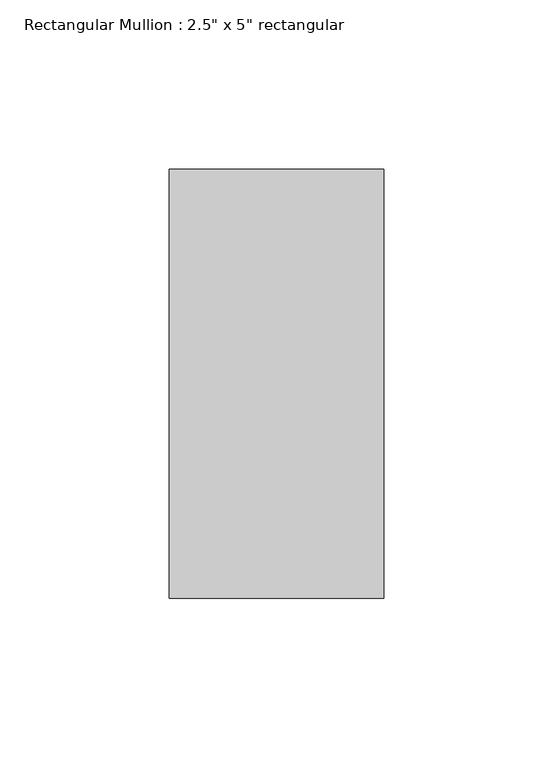
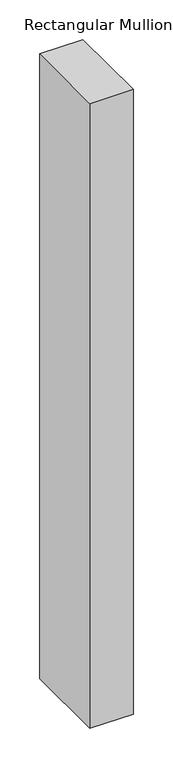
"""IFC4 building model written with IfcOpenShell, lengths in millimetres: member geometry."""

import ifcopenshell
import ifcopenshell.guid

model = None  # the IFC model being written
_history = None  # IfcOwnerHistory: only IFC2X3 demands one
_inside = {}  # id of a spatial element -> (the spatial element, [elements in it])
_under = {}  # id of a project, library or spatial element -> (it, [spatial elements below it])
_declared = {}  # id of a project -> (the project, [libraries it declares])
_typed = {}  # id of a type object -> (the type object, [elements of that type])
_made_of = {}  # id of a material, layer set ... -> (it, [elements and type objects made of it])


def new_model(schema):
    """Start an empty IFC model of exactly this schema.

    Asked for "IFC4X3", IfcOpenShell would pick the latest addendum, in which some entities
    have other attributes; the version numbers below select the first issue.
    IFC2X3 requires an IfcOwnerHistory on every rooted entity: one is made here for all.
    """
    global model, _history
    if schema == "IFC4X3":
        model = ifcopenshell.file(schema_version=(4, 3, 0, 0))
    else:
        model = ifcopenshell.file(schema=schema)
    _inside.clear()
    _under.clear()
    _declared.clear()
    _typed.clear()
    _made_of.clear()
    _history = None
    if model.schema == "IFC2X3":
        org = make("IfcOrganization", Name="unknown")
        user = make(
            "IfcPersonAndOrganization",
            ThePerson=make("IfcPerson", FamilyName="unknown"),
            TheOrganization=org,
        )
        app = make(
            "IfcApplication",
            ApplicationDeveloper=org,
            Version="unknown",
            ApplicationFullName="unknown",
            ApplicationIdentifier="unknown",
        )
        _history = make(
            "IfcOwnerHistory",
            OwningUser=user,
            OwningApplication=app,
            ChangeAction="ADDED",
            CreationDate=0,
        )
    return model


def make(cls, **values):
    """One entity of the class cls with the attributes given. An attribute that is None is left unset."""
    return model.create_entity(
        cls, **{name: value for name, value in values.items() if value is not None}
    )


def rooted(cls, **values):
    """An entity with a GlobalId (a new one), such as an element, a storey or a relation."""
    return make(cls, GlobalId=ifcopenshell.guid.new(), OwnerHistory=_history, **values)


def si_unit(unit_type, name, prefix=None):
    """IfcSIUnit, for example si_unit("LENGTHUNIT", "METRE", prefix="MILLI")."""
    return make("IfcSIUnit", UnitType=unit_type, Prefix=prefix, Name=name)


def assignment(units):
    """IfcUnitAssignment: the units of a project."""
    return None if units is None else make("IfcUnitAssignment", Units=units)


def point(xyz):
    """IfcCartesianPoint."""
    return None if xyz is None else make("IfcCartesianPoint", Coordinates=xyz)


def direction(xyz):
    """IfcDirection."""
    return None if xyz is None else make("IfcDirection", DirectionRatios=xyz)


def frame(location, z_axis=None, x_axis=None):
    """IfcAxis2Placement3D, a coordinate frame: its origin and axes. An axis left out is left unset."""
    return make(
        "IfcAxis2Placement3D",
        Location=point(location),
        Axis=direction(z_axis),
        RefDirection=direction(x_axis),
    )


def origin():
    """The frame at (0, 0, 0) with its axes left unset."""
    return frame((0.0, 0.0, 0.0))


def place(relative_to, where):
    """IfcLocalPlacement: puts the frame where relative to a parent placement (None: the world)."""
    return make(
        "IfcLocalPlacement", PlacementRelTo=relative_to, RelativePlacement=where
    )


def context(
    kind, dimensions, precision=None, world=None, true_north=None, identifier=None
):
    """IfcGeometricRepresentationContext, for example the 3D "Model" context."""
    return make(
        "IfcGeometricRepresentationContext",
        ContextIdentifier=identifier,
        ContextType=kind,
        CoordinateSpaceDimension=dimensions,
        Precision=precision,
        WorldCoordinateSystem=world,
        TrueNorth=true_north,
    )


def project(units=None, contexts=None):
    """IfcProject with its units and contexts."""
    return rooted(
        "IfcProject",
        Name="project",
        RepresentationContexts=contexts,
        UnitsInContext=assignment(units),
    )


def spatial(cls, under=None, at=None, **own):
    """A site, building, storey or space (cls), placed at a placement, below another one or the project."""
    s = rooted(cls, ObjectPlacement=at, **own)
    if under is not None:
        _under.setdefault(under.id(), (under, []))[1].append(s)
    return s


def polyline(points):
    """IfcPolyline through the points."""
    return make("IfcPolyline", Points=[point(p) for p in points])


def outline(outer, holes=None, kind="AREA"):
    """IfcArbitraryClosedProfileDef: a profile drawn as a closed curve; with holes, ...WithVoids."""
    if holes is None:
        return make("IfcArbitraryClosedProfileDef", ProfileType=kind, OuterCurve=outer)
    return make(
        "IfcArbitraryProfileDefWithVoids",
        ProfileType=kind,
        OuterCurve=outer,
        InnerCurves=holes,
    )


def extrude(swept, where, along, depth):
    """IfcExtrudedAreaSolid: the profile swept, set in the frame where, extruded along a direction by depth."""
    return make(
        "IfcExtrudedAreaSolid",
        SweptArea=swept,
        Position=where,
        ExtrudedDirection=direction(along),
        Depth=depth,
    )


def shape(context_of_items, identifier, shape_type, items):
    """IfcShapeRepresentation: the items that make up one representation, for example the "Body"."""
    return make(
        "IfcShapeRepresentation",
        ContextOfItems=context_of_items,
        RepresentationIdentifier=identifier,
        RepresentationType=shape_type,
        Items=items,
    )


def source(mapping_origin, context_of_items, identifier, shape_type, items):
    """IfcRepresentationMap: a shape defined once, which mapped items show again and again."""
    return make(
        "IfcRepresentationMap",
        MappingOrigin=mapping_origin,
        MappedRepresentation=shape(context_of_items, identifier, shape_type, items),
    )


def transform(
    local_origin,
    x_axis=None,
    y_axis=None,
    z_axis=None,
    scale=None,
    scale2=None,
    scale3=None,
    uniform=True,
):
    """IfcCartesianTransformationOperator3D, or its non-uniform kind. x_axis, y_axis, z_axis: its Axis1, 2, 3."""
    if uniform:
        return make(
            "IfcCartesianTransformationOperator3D",
            Axis1=direction(x_axis),
            Axis2=direction(y_axis),
            LocalOrigin=point(local_origin),
            Scale=scale,
            Axis3=direction(z_axis),
        )
    return make(
        "IfcCartesianTransformationOperator3DnonUniform",
        Axis1=direction(x_axis),
        Axis2=direction(y_axis),
        LocalOrigin=point(local_origin),
        Scale=scale,
        Axis3=direction(z_axis),
        Scale2=scale2,
        Scale3=scale3,
    )


def mapped(mapping_source, mapping_target):
    """IfcMappedItem: shows the shape of a source again, moved by a transform."""
    return make(
        "IfcMappedItem", MappingSource=mapping_source, MappingTarget=mapping_target
    )


def made_of(thing, what):
    """Note that an element or type object is made of a material, layer set ...; save() writes the relation."""
    if what is not None:
        _made_of.setdefault(what.id(), (what, []))[1].append(thing)
    return thing


def element(
    cls,
    number,
    at=None,
    inside=None,
    cuts=None,
    type_object=None,
    material=None,
    context=None,
    identifier="Body",
    shape_type=None,
    held_by="IfcProductDefinitionShape",
    body=None,
    shapes=None,
    **own,
):
    """One element of the class cls, such as IfcWall. Its Tag is "e" and its number.

    at: its placement. inside: the storey or other place that contains it. cuts: it is an
    opening in that element (IfcRelVoidsElement). A single representation is given by context,
    identifier, shape_type and body (its items); several are given by shapes. held_by: the class
    of the entity that holds the representations. save() writes the other relations.
    """
    e = rooted(cls, Tag="e%d" % number, ObjectPlacement=at, **own)
    if body is not None:
        shapes = [shape(context, identifier, shape_type, body)]
    if shapes is not None:
        e.Representation = make(held_by, Representations=shapes)
    if inside is not None:
        _inside.setdefault(inside.id(), (inside, []))[1].append(e)
    if cuts is not None:
        rooted(
            "IfcRelVoidsElement", RelatingBuildingElement=cuts, RelatedOpeningElement=e
        )
    if type_object is not None:
        _typed.setdefault(type_object.id(), (type_object, []))[1].append(e)
    return made_of(e, material)


def aggregate(whole, parts):
    """IfcRelAggregates: a whole, such as a stair, and the parts it consists of."""
    return rooted("IfcRelAggregates", RelatingObject=whole, RelatedObjects=parts)


def save(model, path):
    """Write the relations noted so far, then the file.

    IfcRelAggregates (storeys below a building ...), IfcRelContainedInSpatialStructure (elements
    in a storey), IfcRelDefinesByType, IfcRelAssociatesMaterial and IfcRelDeclares: one each for
    every whole, place, type object, material and project.
    """
    for whole, parts in _under.values():
        aggregate(whole, parts)
    for where, things in _inside.values():
        rooted(
            "IfcRelContainedInSpatialStructure",
            RelatedElements=things,
            RelatingStructure=where,
        )
    for kind, things in _typed.values():
        rooted("IfcRelDefinesByType", RelatedObjects=things, RelatingType=kind)
    for what, things in _made_of.values():
        rooted("IfcRelAssociatesMaterial", RelatedObjects=things, RelatingMaterial=what)
    for by, libraries in _declared.values():
        rooted("IfcRelDeclares", RelatingContext=by, RelatedDefinitions=libraries)
    model.write(path)


def member_1f3bd77c(model_context):
    return source(origin(), model_context, "Body", "SweptSolid", [
        extrude(outline(polyline([(0.0, 63.5), (0.0, -63.5), (-63.5, -63.5), (-63.5, 63.5), (0.0, 63.5)])), frame((0.0, 0.0, -965.1999998), z_axis=(0.0, 0.0, 1.0), x_axis=(1.0, 0.0, 0.0)), (0.0, 0.0, 1.0), 965.1999998),
    ])


if __name__ == "__main__":
    model = new_model("IFC4")
    model_context = context("Model", 3, world=origin())
    ifc_project = project(units=[si_unit("LENGTHUNIT", "METRE", prefix="MILLI")], contexts=[model_context])
    site = spatial("IfcSite", under=ifc_project)
    building = spatial("IfcBuilding", under=site)
    placement = place(None, origin())
    member_shape = member_1f3bd77c(model_context)
    element("IfcMember", 1, ObjectType="Rectangular Mullion : 2.5\" x 5\" rectangular", at=placement, inside=building, context=model_context, shape_type="MappedRepresentation", body=[
        mapped(member_shape, transform((0.0, 0.0, 0.0), x_axis=(1.0, 0.0, 0.0), y_axis=(0.0, 1.0, 0.0), z_axis=(0.0, 0.0, 1.0))),
    ])
    save(model, "model.ifc")

# Revit data of these elements
# Project information
#   Organization Name = "G3B Press"
#   Organization Description = "Paul F. Aubin Cosulting Services, Inc."
#   Building Name = "Revit Essentials for Architecture"
#   Author = "Paul F. Aubin"
#   Author Website = "https://www.paulaubin.com"
#   Copyright = "Copyright © 2020 Paul F Aubin, all rights reserved"
#   Workset = "Project Info"
#   Design Option = "Main Model"
#   Project Issue Date = "8/1/2020"
#   Project Status = "Design Development"
#   Client Name = "Worksharing"
#   Project Address = "123 State ST\nSuite 301\nChicago, IL 60606"
#   Project Name = "WS Commercial"
#   Project Number = "2020.04A"
# Type "Rectangular Mullion : 2.5\" x 5\" rectangular"
#   built-in parameter 1007304 = 0.416667 (stored number, unit not read)
#   built-in parameter 1007301 = 0.104167 (stored number, unit not read)
#   built-in parameter 1007300 = 0.104167 (stored number, unit not read)
# Element 1 (IfcMember, "Rectangular Mullion : 2.5\" x 5\" rectangular")
#   Materials on its faces: "Aluminum"
# Materials
#   "Aluminum": class "Metal", colour RGB 247 247 247, transparency 0, Description = "Aluminum 6061", Cost = 0
